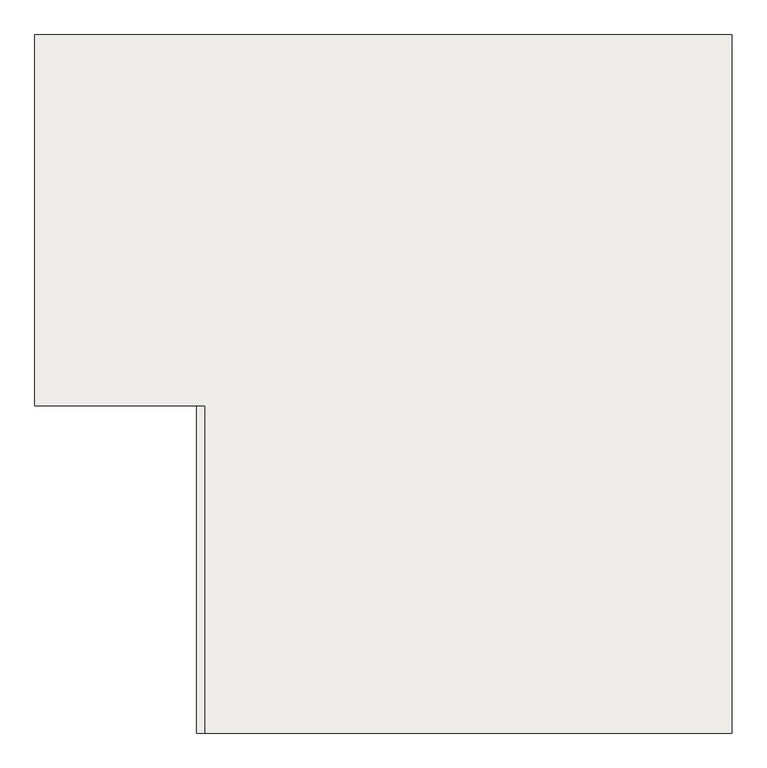
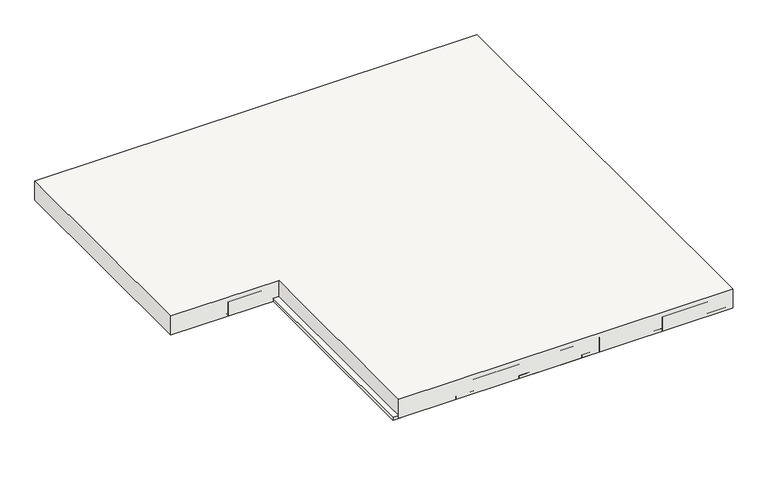
"""IFC4 building model written with IfcOpenShell, lengths in millimetres: slab geometry, Pano 5 (16 cm)."""

from ifc_helpers import new_model, si_unit, origin, origin_with_axes, place, context, project, spatial, polyline, outline, extrude, source, transform, mapped, element, save


def slab_56df2be2(model_context):
    return source(origin(), model_context, "Body", "SweptSolid", [
        extrude(outline(polyline([(2655.0, 4360.0), (2655.0, 840.0), (0.0, 840.0), (0.0, 2490.0), (-860.0, 2490.0), (-860.0, 4360.0), (2655.0, 4360.0)])), origin_with_axes(), (0.0, 0.0, 1.0), 160.0),
        extrude(outline(polyline([(455.0, 3840.0), (95.0, 3840.0), (95.0, 4335.0), (455.0, 4335.0), (455.0, 3840.0)])), origin_with_axes(), (0.0, 0.0, 1.0), 120.0),
        extrude(outline(polyline([(1095.0, 840.0), (955.0, 840.0), (955.0, 4360.0), (1095.0, 4360.0), (1095.0, 840.0)])), origin_with_axes(), (0.0, 0.0, 1.0), 24.0),
        extrude(outline(polyline([(1955.0, 3340.0), (1595.0, 3340.0), (1595.0, 3835.0), (1955.0, 3835.0), (1955.0, 3340.0)])), origin_with_axes(), (0.0, 0.0, 1.0), 120.0),
        extrude(outline(polyline([(955.0, 4340.0), (595.0, 4340.0), (595.0, 4355.0), (955.0, 4355.0), (955.0, 4340.0)])), origin_with_axes(), (0.0, 0.0, 1.0), 120.0),
        extrude(outline(polyline([(1455.0, 4340.0), (1095.0, 4340.0), (1095.0, 4355.0), (1455.0, 4355.0), (1455.0, 4340.0)])), origin_with_axes(), (0.0, 0.0, 1.0), 120.0),
        extrude(outline(polyline([(1955.0, 840.0), (1595.0, 840.0), (1595.0, 1335.0), (1955.0, 1335.0), (1955.0, 840.0)])), origin_with_axes(), (0.0, 0.0, 1.0), 120.0),
        extrude(outline(polyline([(455.0, 2340.0), (95.0, 2340.0), (95.0, 2835.0), (455.0, 2835.0), (455.0, 2340.0)])), origin_with_axes(), (0.0, 0.0, 1.0), 120.0),
        extrude(outline(polyline([(455.0, 2840.0), (95.0, 2840.0), (95.0, 3335.0), (455.0, 3335.0), (455.0, 2840.0)])), origin_with_axes(), (0.0, 0.0, 1.0), 120.0),
        extrude(outline(polyline([(955.0, 2340.0), (595.0, 2340.0), (595.0, 2835.0), (955.0, 2835.0), (955.0, 2340.0)])), origin_with_axes(), (0.0, 0.0, 1.0), 120.0),
        extrude(outline(polyline([(-45.0, 3490.0), (-405.0, 3490.0), (-405.0, 3985.0), (-45.0, 3985.0), (-45.0, 3490.0)])), origin_with_axes(), (0.0, 0.0, 1.0), 120.0),
        extrude(outline(polyline([(2455.0, 3840.0), (2095.0, 3840.0), (2095.0, 4335.0), (2455.0, 4335.0), (2455.0, 3840.0)])), origin_with_axes(), (0.0, 0.0, 1.0), 120.0),
        extrude(outline(polyline([(455.0, 3340.0), (95.0, 3340.0), (95.0, 3835.0), (455.0, 3835.0), (455.0, 3340.0)])), origin_with_axes(), (0.0, 0.0, 1.0), 120.0),
        extrude(outline(polyline([(955.0, 840.0), (595.0, 840.0), (595.0, 1335.0), (955.0, 1335.0), (955.0, 840.0)])), origin_with_axes(), (0.0, 0.0, 1.0), 120.0),
        extrude(outline(polyline([(1455.0, 1340.0), (1095.0, 1340.0), (1095.0, 1835.0), (1455.0, 1835.0), (1455.0, 1340.0)])), origin_with_axes(), (0.0, 0.0, 1.0), 120.0),
        extrude(outline(polyline([(1955.0, 2340.0), (1595.0, 2340.0), (1595.0, 2835.0), (1955.0, 2835.0), (1955.0, 2340.0)])), origin_with_axes(), (0.0, 0.0, 1.0), 120.0),
        extrude(outline(polyline([(2455.0, 3340.0), (2095.0, 3340.0), (2095.0, 3835.0), (2455.0, 3835.0), (2455.0, 3340.0)])), origin_with_axes(), (0.0, 0.0, 1.0), 120.0),
        extrude(outline(polyline([(-45.0, 2490.0), (-405.0, 2490.0), (-405.0, 2985.0), (-45.0, 2985.0), (-45.0, 2490.0)])), origin_with_axes(), (0.0, 0.0, 1.0), 120.0),
        extrude(outline(polyline([(1455.0, 2340.0), (1095.0, 2340.0), (1095.0, 2835.0), (1455.0, 2835.0), (1455.0, 2340.0)])), origin_with_axes(), (0.0, 0.0, 1.0), 120.0),
        extrude(outline(polyline([(2455.0, 1840.0), (2095.0, 1840.0), (2095.0, 2335.0), (2455.0, 2335.0), (2455.0, 1840.0)])), origin_with_axes(), (0.0, 0.0, 1.0), 120.0),
        extrude(outline(polyline([(955.0, 1340.0), (595.0, 1340.0), (595.0, 1835.0), (955.0, 1835.0), (955.0, 1340.0)])), origin_with_axes(), (0.0, 0.0, 1.0), 120.0),
        extrude(outline(polyline([(1955.0, 1840.0), (1595.0, 1840.0), (1595.0, 2335.0), (1955.0, 2335.0), (1955.0, 1840.0)])), origin_with_axes(), (0.0, 0.0, 1.0), 120.0),
        extrude(outline(polyline([(-45.0, 2990.0), (-405.0, 2990.0), (-405.0, 3485.0), (-45.0, 3485.0), (-45.0, 2990.0)])), origin_with_axes(), (0.0, 0.0, 1.0), 120.0),
        extrude(outline(polyline([(955.0, 1840.0), (595.0, 1840.0), (595.0, 2335.0), (955.0, 2335.0), (955.0, 1840.0)])), origin_with_axes(), (0.0, 0.0, 1.0), 120.0),
        extrude(outline(polyline([(2095.0, 840.0), (1955.0, 840.0), (1955.0, 4360.0), (2095.0, 4360.0), (2095.0, 840.0)])), origin_with_axes(), (0.0, 0.0, 1.0), 24.0),
        extrude(outline(polyline([(1455.0, 3840.0), (1095.0, 3840.0), (1095.0, 4335.0), (1455.0, 4335.0), (1455.0, 3840.0)])), origin_with_axes(), (0.0, 0.0, 1.0), 120.0),
        extrude(outline(polyline([(1955.0, 1340.0), (1595.0, 1340.0), (1595.0, 1835.0), (1955.0, 1835.0), (1955.0, 1340.0)])), origin_with_axes(), (0.0, 0.0, 1.0), 120.0),
        extrude(outline(polyline([(1455.0, 2840.0), (1095.0, 2840.0), (1095.0, 3335.0), (1455.0, 3335.0), (1455.0, 2840.0)])), origin_with_axes(), (0.0, 0.0, 1.0), 120.0),
        extrude(outline(polyline([(2455.0, 2340.0), (2095.0, 2340.0), (2095.0, 2835.0), (2455.0, 2835.0), (2455.0, 2340.0)])), origin_with_axes(), (0.0, 0.0, 1.0), 120.0),
        extrude(outline(polyline([(1955.0, 3840.0), (1595.0, 3840.0), (1595.0, 4335.0), (1955.0, 4335.0), (1955.0, 3840.0)])), origin_with_axes(), (0.0, 0.0, 1.0), 120.0),
        extrude(outline(polyline([(455.0, 840.0), (95.0, 840.0), (95.0, 1335.0), (455.0, 1335.0), (455.0, 840.0)])), origin_with_axes(), (0.0, 0.0, 1.0), 120.0),
        extrude(outline(polyline([(2455.0, 1340.0), (2095.0, 1340.0), (2095.0, 1835.0), (2455.0, 1835.0), (2455.0, 1340.0)])), origin_with_axes(), (0.0, 0.0, 1.0), 120.0),
        extrude(outline(polyline([(955.0, 3840.0), (595.0, 3840.0), (595.0, 4335.0), (955.0, 4335.0), (955.0, 3840.0)])), origin_with_axes(), (0.0, 0.0, 1.0), 120.0),
        extrude(outline(polyline([(-405.0, 2490.0), (-545.0, 2490.0), (-545.0, 4360.0), (-405.0, 4360.0), (-405.0, 2490.0)])), origin_with_axes(), (0.0, 0.0, 1.0), 24.0),
        extrude(outline(polyline([(455.0, 1840.0), (95.0, 1840.0), (95.0, 2335.0), (455.0, 2335.0), (455.0, 1840.0)])), origin_with_axes(), (0.0, 0.0, 1.0), 120.0),
        extrude(outline(polyline([(955.0, 2840.0), (595.0, 2840.0), (595.0, 3335.0), (955.0, 3335.0), (955.0, 2840.0)])), origin_with_axes(), (0.0, 0.0, 1.0), 120.0),
        extrude(outline(polyline([(2455.0, 4340.0), (2095.0, 4340.0), (2095.0, 4355.0), (2455.0, 4355.0), (2455.0, 4340.0)])), origin_with_axes(), (0.0, 0.0, 1.0), 120.0),
        extrude(outline(polyline([(-45.0, 3990.0), (-405.0, 3990.0), (-405.0, 4355.0), (-45.0, 4355.0), (-45.0, 3990.0)])), origin_with_axes(), (0.0, 0.0, 1.0), 120.0),
        extrude(outline(polyline([(955.0, 3340.0), (595.0, 3340.0), (595.0, 3835.0), (955.0, 3835.0), (955.0, 3340.0)])), origin_with_axes(), (0.0, 0.0, 1.0), 120.0),
        extrude(outline(polyline([(1455.0, 1840.0), (1095.0, 1840.0), (1095.0, 2335.0), (1455.0, 2335.0), (1455.0, 1840.0)])), origin_with_axes(), (0.0, 0.0, 1.0), 120.0),
        extrude(outline(polyline([(1955.0, 2840.0), (1595.0, 2840.0), (1595.0, 3335.0), (1955.0, 3335.0), (1955.0, 2840.0)])), origin_with_axes(), (0.0, 0.0, 1.0), 120.0),
        extrude(outline(polyline([(455.0, 1340.0), (95.0, 1340.0), (95.0, 1835.0), (455.0, 1835.0), (455.0, 1340.0)])), origin_with_axes(), (0.0, 0.0, 1.0), 120.0),
        extrude(outline(polyline([(2595.0, 840.0), (2455.0, 840.0), (2455.0, 4360.0), (2595.0, 4360.0), (2595.0, 840.0)])), origin_with_axes(), (0.0, 0.0, 1.0), 24.0),
        extrude(outline(polyline([(455.0, 4340.0), (95.0, 4340.0), (95.0, 4355.0), (455.0, 4355.0), (455.0, 4340.0)])), origin_with_axes(), (0.0, 0.0, 1.0), 120.0),
        extrude(outline(polyline([(2455.0, 2840.0), (2095.0, 2840.0), (2095.0, 3335.0), (2455.0, 3335.0), (2455.0, 2840.0)])), origin_with_axes(), (0.0, 0.0, 1.0), 120.0),
        extrude(outline(polyline([(1455.0, 3340.0), (1095.0, 3340.0), (1095.0, 3835.0), (1455.0, 3835.0), (1455.0, 3340.0)])), origin_with_axes(), (0.0, 0.0, 1.0), 120.0),
        extrude(outline(polyline([(595.0, 840.0), (455.0, 840.0), (455.0, 4360.0), (595.0, 4360.0), (595.0, 840.0)])), origin_with_axes(), (0.0, 0.0, 1.0), 24.0),
        extrude(outline(polyline([(2455.0, 840.0), (2095.0, 840.0), (2095.0, 1335.0), (2455.0, 1335.0), (2455.0, 840.0)])), origin_with_axes(), (0.0, 0.0, 1.0), 120.0),
        extrude(outline(polyline([(1595.0, 840.0), (1455.0, 840.0), (1455.0, 4360.0), (1595.0, 4360.0), (1595.0, 840.0)])), origin_with_axes(), (0.0, 0.0, 1.0), 24.0),
        extrude(outline(polyline([(95.0, 840.0), (-45.0, 840.0), (-45.0, 4360.0), (95.0, 4360.0), (95.0, 840.0)])), origin_with_axes(), (0.0, 0.0, 1.0), 24.0),
        extrude(outline(polyline([(1955.0, 4340.0), (1595.0, 4340.0), (1595.0, 4355.0), (1955.0, 4355.0), (1955.0, 4340.0)])), origin_with_axes(), (0.0, 0.0, 1.0), 120.0),
        extrude(outline(polyline([(1455.0, 840.0), (1095.0, 840.0), (1095.0, 1335.0), (1455.0, 1335.0), (1455.0, 840.0)])), origin_with_axes(), (0.0, 0.0, 1.0), 120.0),
    ])


if __name__ == "__main__":
    model = new_model("IFC4")
    model_context = context("Model", 3, world=origin())
    ifc_project = project(units=[si_unit("LENGTHUNIT", "METRE", prefix="MILLI")], contexts=[model_context])
    site = spatial("IfcSite", under=ifc_project)
    building = spatial("IfcBuilding", under=site)
    placement = place(None, origin())
    slab_shape = slab_56df2be2(model_context)
    element("IfcSlab", 1, ObjectType="Pano 5 (16 cm)", at=placement, inside=building, context=model_context, shape_type="MappedRepresentation", body=[
        mapped(slab_shape, transform((0.0, 0.0, 0.0), x_axis=(1.0, 0.0, 0.0), y_axis=(0.0, 1.0, 0.0), z_axis=(0.0, 0.0, 1.0))),
    ])
    save(model, "model.ifc")

# Revit data of these elements
# Element 1 (IfcSlab, "Pano 5 (16 cm)")
#   Materials on its faces: "Molde de poliestireno", "Concreto armado", "RGB 168-169-158"
# Materials
#   "Molde de poliestireno": class "Não atribuído", colour RGB 255 255 255, transparency 0
#   "Concreto armado": class "Não atribuído", colour RGB 168 169 158, transparency 0
#   "RGB 168-169-158": class "Não atribuído", colour RGB 168 169 158, transparency 0
